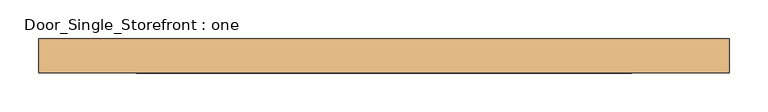
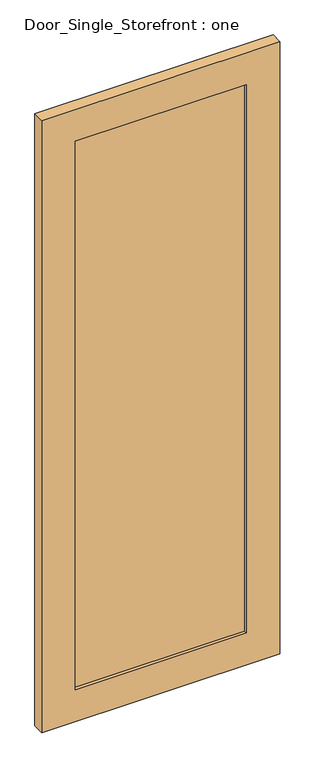
"""IFC4 building model written with IfcOpenShell, lengths in millimetres: door geometry, Door_Single_Storefront : one."""

from ifc_helpers import new_model, si_unit, frame, origin, place, context, project, spatial, polyline, outline, extrude, source, transform, mapped, element, save


def door_single_storefront_one_e8b64d58(model_context):
    return source(origin(), model_context, "Body", "SweptSolid", [
        extrude(outline(polyline([(321.46875, 6.35), (321.46875, -12.7), (-321.46875, -12.7), (-321.46875, 6.35), (321.46875, 6.35)])), frame((0.0, 0.0, 127.0), z_axis=(0.0, 0.0, 1.0), x_axis=(1.0, 0.0, 0.0)), (0.0, 0.0, 1.0), 2184.4),
        extrude(outline(polyline([(2438.4, -448.46875), (0.0, -448.46875), (0.0, 448.46875), (2438.4, 448.46875), (2438.4, -448.46875)]), holes=[polyline([(127.0, 321.46875), (127.0, -321.46875), (2311.4, -321.46875), (2311.4, 321.46875), (127.0, 321.46875)])]), frame((0.0, -25.4, 0.0), z_axis=(0.0, 1.0, 0.0), x_axis=(0.0, 0.0, 1.0)), (0.0, 0.0, 1.0), 44.45),
    ])


if __name__ == "__main__":
    model = new_model("IFC4")
    model_context = context("Model", 3, world=origin())
    ifc_project = project(units=[si_unit("LENGTHUNIT", "METRE", prefix="MILLI")], contexts=[model_context])
    site = spatial("IfcSite", under=ifc_project)
    building = spatial("IfcBuilding", under=site)
    placement = place(None, origin())
    door_single_storefront_one_shape = door_single_storefront_one_e8b64d58(model_context)
    element("IfcDoor", 1, ObjectType="Door_Single_Storefront : one", at=placement, inside=building, context=model_context, shape_type="MappedRepresentation", body=[
        mapped(door_single_storefront_one_shape, transform((0.0, 0.0, 0.0), x_axis=(1.0, 0.0, 0.0), y_axis=(0.0, 1.0, 0.0), z_axis=(0.0, 0.0, 1.0))),
    ])
    save(model, "model.ifc")

# Revit data of these elements
# Type "Door_Single_Storefront : one"
#   Type Mark = "27"
#   Analytic Construction = "<None>"
#   Stile_Width = 0' - 5"
#   Door_Thickness = 0' - 1 3/4"
#   Door_Offset = 0' - 1"
#   Glass_Material = SAFETY GLAZING
#   Frame_Material = INTERIOR GRADE ALUMINUM STOREFRONT W/ SAFETY GLAZING
#   Function = (empty or 0)
# Element 1 (IfcDoor, "Door_Single_Storefront : one")
#   Materials on its faces: "INTERIOR GRADE ALUMINUM STOREFRONT W/ SAFETY GLAZING", "SAFETY GLAZING"
# Materials
#   "SAFETY GLAZING": class "Glass", colour RGB 142 168 196, transparency 0.75, Description = "Soda Lime Glass", Cost = 0
#   "INTERIOR GRADE ALUMINUM STOREFRONT W/ SAFETY GLAZING": class "Metal", colour RGB 226 226 226, transparency 0, Description = "Aluminum 6061", Cost = 0
